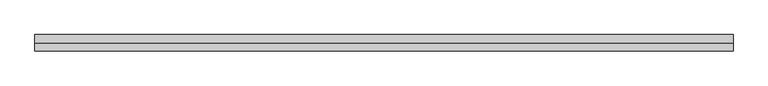
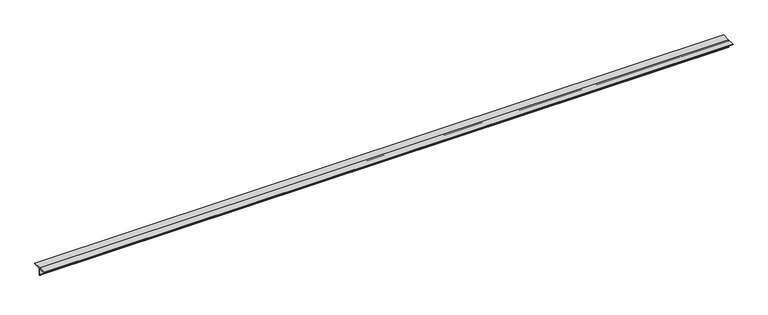
"""IFC4 building model written with IfcOpenShell, lengths in millimetres: member geometry, 0123_Steel Framing_2Ls-KSD3502 : H_SB_AR_S03_2Ls-130x130x12_HBR1."""

from ifc_helpers import new_model, si_unit, point, frame, frame_2d, origin, place, context, project, spatial, polyline, circle_curve, trimmed, segment, composite_curve, outline, extrude, source, transform, mapped, element, save


def member_b0bd77dc(model_context):
    return source(origin(), model_context, "Body", "SweptSolid", [
        extrude(outline(composite_curve([segment(polyline([(0.0, 36.4), (130.0, 36.4)]), True, "CONTINUOUS"), segment(trimmed(circle_curve(frame_2d((118.0, 36.4)), 12.0), [point((130.0, 36.4))], [point((118.0, 24.4))], False, "CARTESIAN"), True, "CONTINUOUS"), segment(polyline([(118.0, 24.4), (24.0, 24.4)]), True, "CONTINUOUS"), segment(trimmed(circle_curve(frame_2d((24.0, 12.4)), 12.0), [point((24.0, 24.4))], [point((12.0, 12.4))], True, "CARTESIAN"), True, "CONTINUOUS"), segment(polyline([(12.0, 12.4), (12.0, -81.6)]), True, "CONTINUOUS"), segment(trimmed(circle_curve(frame_2d((0.0, -81.6)), 12.0), [point((12.0, -81.6))], [point((0.0, -93.6))], False, "CARTESIAN"), True, "CONTINUOUS"), segment(polyline([(0.0, -93.6), (0.0, 36.4)]), True, "CONTINUOUS")], self_intersect=False)), frame((-5571.7417611, 0.0, 0.0), z_axis=(1.0, 0.0, 0.0), x_axis=(0.0, 1.0, 0.0)), (0.0, 0.0, 1.0), 11162.5198652),
        extrude(outline(composite_curve([segment(polyline([(0.0, 36.4), (0.0, -93.6)]), True, "CONTINUOUS"), segment(trimmed(circle_curve(frame_2d((0.0, -81.6)), 12.0), [point((0.0, -93.6))], [point((-12.0, -81.6))], False, "CARTESIAN"), True, "CONTINUOUS"), segment(polyline([(-12.0, -81.6), (-12.0, 12.4)]), True, "CONTINUOUS"), segment(trimmed(circle_curve(frame_2d((-24.0, 12.4)), 12.0), [point((-12.0, 12.4))], [point((-24.0, 24.4))], True, "CARTESIAN"), True, "CONTINUOUS"), segment(polyline([(-24.0, 24.4), (-118.0, 24.4)]), True, "CONTINUOUS"), segment(trimmed(circle_curve(frame_2d((-118.0, 36.4)), 12.0), [point((-118.0, 24.4))], [point((-130.0, 36.4))], False, "CARTESIAN"), True, "CONTINUOUS"), segment(polyline([(-130.0, 36.4), (0.0, 36.4)]), True, "CONTINUOUS")], self_intersect=False)), frame((-5571.7417611, 0.0, 0.0), z_axis=(1.0, 0.0, 0.0), x_axis=(0.0, 1.0, 0.0)), (0.0, 0.0, 1.0), 11162.5198652),
    ])


if __name__ == "__main__":
    model = new_model("IFC4")
    model_context = context("Model", 3, world=origin())
    ifc_project = project(units=[si_unit("LENGTHUNIT", "METRE", prefix="MILLI")], contexts=[model_context])
    site = spatial("IfcSite", under=ifc_project)
    building = spatial("IfcBuilding", under=site)
    placement = place(None, origin())
    member_shape = member_b0bd77dc(model_context)
    element("IfcMember", 1, ObjectType="0123_Steel Framing_2Ls-KSD3502 : H_SB_AR_S03_2Ls-130x130x12_HBR1", at=placement, inside=building, context=model_context, shape_type="MappedRepresentation", body=[
        mapped(member_shape, transform((0.0, 0.0, 0.0), x_axis=(1.0, 0.0, 0.0), y_axis=(0.0, 1.0, 0.0), z_axis=(0.0, 0.0, 1.0))),
    ])
    save(model, "model.ifc")

# Revit data of these elements
# Type "0123_Steel Framing_2Ls-KSD3502 : H_SB_AR_S03_2Ls-130x130x12_HBR1"
#   Type Mark = "HBR1"
#   Assembly Code = "B10"
#   Legs = "SLBB"
#   W = 8.97
#   Perimeter = 1.04 m²/m
#   Nominal Weight = 46.80 kgf/m
#   Length [instance default] = 1000 mm
#   Space = 0 mm
#   b = 130 mm
#   d = 130 mm
#   t = 12 mm
#   y = 36.4 mm
#   A = 0.005952 m²
#   Structural Material [instance default] = Steel ASTM A36
# Element 1 (IfcMember, "0123_Steel Framing_2Ls-KSD3502 : H_SB_AR_S03_2Ls-130x130x12_HBR1")
#   Materials on its faces: "Steel ASTM A36"
# Materials
#   "Steel ASTM A36": class "Metal", colour RGB 199 199 199, transparency 0, Description = "Structural steel, ASTM A36 Grade B, mill finish", Cost = 0
